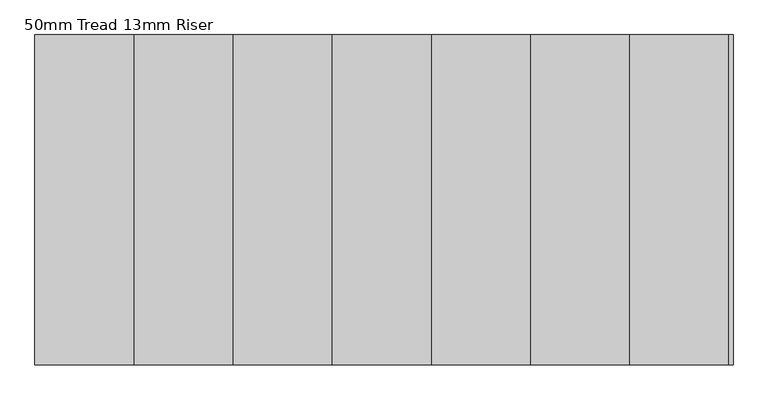
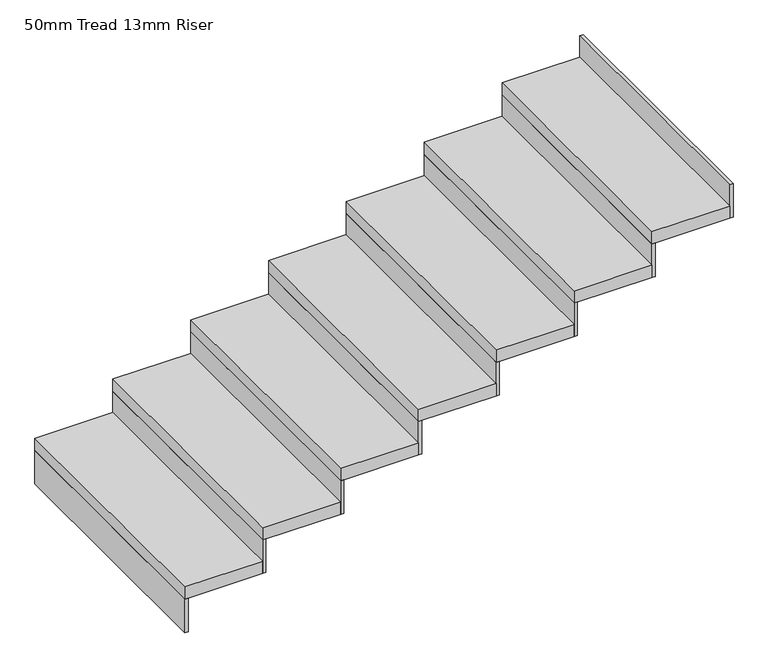
"""IFC4 building model written with IfcOpenShell, lengths in millimetres: stair flight geometry, 50mm Tread 13mm Riser."""

import ifcopenshell
import ifcopenshell.guid

model = None  # the IFC model being written
_history = None  # IfcOwnerHistory: only IFC2X3 demands one
_inside = {}  # id of a spatial element -> (the spatial element, [elements in it])
_under = {}  # id of a project, library or spatial element -> (it, [spatial elements below it])
_declared = {}  # id of a project -> (the project, [libraries it declares])
_typed = {}  # id of a type object -> (the type object, [elements of that type])
_made_of = {}  # id of a material, layer set ... -> (it, [elements and type objects made of it])


def new_model(schema):
    """Start an empty IFC model of exactly this schema.

    Asked for "IFC4X3", IfcOpenShell would pick the latest addendum, in which some entities
    have other attributes; the version numbers below select the first issue.
    IFC2X3 requires an IfcOwnerHistory on every rooted entity: one is made here for all.
    """
    global model, _history
    if schema == "IFC4X3":
        model = ifcopenshell.file(schema_version=(4, 3, 0, 0))
    else:
        model = ifcopenshell.file(schema=schema)
    _inside.clear()
    _under.clear()
    _declared.clear()
    _typed.clear()
    _made_of.clear()
    _history = None
    if model.schema == "IFC2X3":
        org = make("IfcOrganization", Name="unknown")
        user = make(
            "IfcPersonAndOrganization",
            ThePerson=make("IfcPerson", FamilyName="unknown"),
            TheOrganization=org,
        )
        app = make(
            "IfcApplication",
            ApplicationDeveloper=org,
            Version="unknown",
            ApplicationFullName="unknown",
            ApplicationIdentifier="unknown",
        )
        _history = make(
            "IfcOwnerHistory",
            OwningUser=user,
            OwningApplication=app,
            ChangeAction="ADDED",
            CreationDate=0,
        )
    return model


def make(cls, **values):
    """One entity of the class cls with the attributes given. An attribute that is None is left unset."""
    return model.create_entity(
        cls, **{name: value for name, value in values.items() if value is not None}
    )


def rooted(cls, **values):
    """An entity with a GlobalId (a new one), such as an element, a storey or a relation."""
    return make(cls, GlobalId=ifcopenshell.guid.new(), OwnerHistory=_history, **values)


def si_unit(unit_type, name, prefix=None):
    """IfcSIUnit, for example si_unit("LENGTHUNIT", "METRE", prefix="MILLI")."""
    return make("IfcSIUnit", UnitType=unit_type, Prefix=prefix, Name=name)


def assignment(units):
    """IfcUnitAssignment: the units of a project."""
    return None if units is None else make("IfcUnitAssignment", Units=units)


def point(xyz):
    """IfcCartesianPoint."""
    return None if xyz is None else make("IfcCartesianPoint", Coordinates=xyz)


def direction(xyz):
    """IfcDirection."""
    return None if xyz is None else make("IfcDirection", DirectionRatios=xyz)


def frame(location, z_axis=None, x_axis=None):
    """IfcAxis2Placement3D, a coordinate frame: its origin and axes. An axis left out is left unset."""
    return make(
        "IfcAxis2Placement3D",
        Location=point(location),
        Axis=direction(z_axis),
        RefDirection=direction(x_axis),
    )


def origin():
    """The frame at (0, 0, 0) with its axes left unset."""
    return frame((0.0, 0.0, 0.0))


def place(relative_to, where):
    """IfcLocalPlacement: puts the frame where relative to a parent placement (None: the world)."""
    return make(
        "IfcLocalPlacement", PlacementRelTo=relative_to, RelativePlacement=where
    )


def context(
    kind, dimensions, precision=None, world=None, true_north=None, identifier=None
):
    """IfcGeometricRepresentationContext, for example the 3D "Model" context."""
    return make(
        "IfcGeometricRepresentationContext",
        ContextIdentifier=identifier,
        ContextType=kind,
        CoordinateSpaceDimension=dimensions,
        Precision=precision,
        WorldCoordinateSystem=world,
        TrueNorth=true_north,
    )


def project(units=None, contexts=None):
    """IfcProject with its units and contexts."""
    return rooted(
        "IfcProject",
        Name="project",
        RepresentationContexts=contexts,
        UnitsInContext=assignment(units),
    )


def spatial(cls, under=None, at=None, **own):
    """A site, building, storey or space (cls), placed at a placement, below another one or the project."""
    s = rooted(cls, ObjectPlacement=at, **own)
    if under is not None:
        _under.setdefault(under.id(), (under, []))[1].append(s)
    return s


def polyline(points):
    """IfcPolyline through the points."""
    return make("IfcPolyline", Points=[point(p) for p in points])


def outline(outer, holes=None, kind="AREA"):
    """IfcArbitraryClosedProfileDef: a profile drawn as a closed curve; with holes, ...WithVoids."""
    if holes is None:
        return make("IfcArbitraryClosedProfileDef", ProfileType=kind, OuterCurve=outer)
    return make(
        "IfcArbitraryProfileDefWithVoids",
        ProfileType=kind,
        OuterCurve=outer,
        InnerCurves=holes,
    )


def extrude(swept, where, along, depth):
    """IfcExtrudedAreaSolid: the profile swept, set in the frame where, extruded along a direction by depth."""
    return make(
        "IfcExtrudedAreaSolid",
        SweptArea=swept,
        Position=where,
        ExtrudedDirection=direction(along),
        Depth=depth,
    )


def shape(context_of_items, identifier, shape_type, items):
    """IfcShapeRepresentation: the items that make up one representation, for example the "Body"."""
    return make(
        "IfcShapeRepresentation",
        ContextOfItems=context_of_items,
        RepresentationIdentifier=identifier,
        RepresentationType=shape_type,
        Items=items,
    )


def source(mapping_origin, context_of_items, identifier, shape_type, items):
    """IfcRepresentationMap: a shape defined once, which mapped items show again and again."""
    return make(
        "IfcRepresentationMap",
        MappingOrigin=mapping_origin,
        MappedRepresentation=shape(context_of_items, identifier, shape_type, items),
    )


def transform(
    local_origin,
    x_axis=None,
    y_axis=None,
    z_axis=None,
    scale=None,
    scale2=None,
    scale3=None,
    uniform=True,
):
    """IfcCartesianTransformationOperator3D, or its non-uniform kind. x_axis, y_axis, z_axis: its Axis1, 2, 3."""
    if uniform:
        return make(
            "IfcCartesianTransformationOperator3D",
            Axis1=direction(x_axis),
            Axis2=direction(y_axis),
            LocalOrigin=point(local_origin),
            Scale=scale,
            Axis3=direction(z_axis),
        )
    return make(
        "IfcCartesianTransformationOperator3DnonUniform",
        Axis1=direction(x_axis),
        Axis2=direction(y_axis),
        LocalOrigin=point(local_origin),
        Scale=scale,
        Axis3=direction(z_axis),
        Scale2=scale2,
        Scale3=scale3,
    )


def mapped(mapping_source, mapping_target):
    """IfcMappedItem: shows the shape of a source again, moved by a transform."""
    return make(
        "IfcMappedItem", MappingSource=mapping_source, MappingTarget=mapping_target
    )


def made_of(thing, what):
    """Note that an element or type object is made of a material, layer set ...; save() writes the relation."""
    if what is not None:
        _made_of.setdefault(what.id(), (what, []))[1].append(thing)
    return thing


def element(
    cls,
    number,
    at=None,
    inside=None,
    cuts=None,
    type_object=None,
    material=None,
    context=None,
    identifier="Body",
    shape_type=None,
    held_by="IfcProductDefinitionShape",
    body=None,
    shapes=None,
    **own,
):
    """One element of the class cls, such as IfcWall. Its Tag is "e" and its number.

    at: its placement. inside: the storey or other place that contains it. cuts: it is an
    opening in that element (IfcRelVoidsElement). A single representation is given by context,
    identifier, shape_type and body (its items); several are given by shapes. held_by: the class
    of the entity that holds the representations. save() writes the other relations.
    """
    e = rooted(cls, Tag="e%d" % number, ObjectPlacement=at, **own)
    if body is not None:
        shapes = [shape(context, identifier, shape_type, body)]
    if shapes is not None:
        e.Representation = make(held_by, Representations=shapes)
    if inside is not None:
        _inside.setdefault(inside.id(), (inside, []))[1].append(e)
    if cuts is not None:
        rooted(
            "IfcRelVoidsElement", RelatingBuildingElement=cuts, RelatedOpeningElement=e
        )
    if type_object is not None:
        _typed.setdefault(type_object.id(), (type_object, []))[1].append(e)
    return made_of(e, material)


def aggregate(whole, parts):
    """IfcRelAggregates: a whole, such as a stair, and the parts it consists of."""
    return rooted("IfcRelAggregates", RelatingObject=whole, RelatedObjects=parts)


def save(model, path):
    """Write the relations noted so far, then the file.

    IfcRelAggregates (storeys below a building ...), IfcRelContainedInSpatialStructure (elements
    in a storey), IfcRelDefinesByType, IfcRelAssociatesMaterial and IfcRelDeclares: one each for
    every whole, place, type object, material and project.
    """
    for whole, parts in _under.values():
        aggregate(whole, parts)
    for where, things in _inside.values():
        rooted(
            "IfcRelContainedInSpatialStructure",
            RelatedElements=things,
            RelatingStructure=where,
        )
    for kind, things in _typed.values():
        rooted("IfcRelDefinesByType", RelatedObjects=things, RelatingType=kind)
    for what, things in _made_of.values():
        rooted("IfcRelAssociatesMaterial", RelatedObjects=things, RelatingMaterial=what)
    for by, libraries in _declared.values():
        rooted("IfcRelDeclares", RelatingContext=by, RelatedDefinitions=libraries)
    model.write(path)


def stair_flight_50mm_tread_13mm_riser_0255b1fd(model_context):
    return source(origin(), model_context, "Body", "SweptSolid", [
        extrude(outline(polyline([(-12593.4172363, -3171.6396273), (-12605.9172363, -3171.6396273), (-12605.9172363, -2171.6396273), (-12593.4172363, -2171.6396273), (-12593.4172363, -3171.6396273)])), frame((0.0, 0.0, 1859.0909091), z_axis=(0.0, 0.0, 1.0), x_axis=(1.0, 0.0, 0.0)), (0.0, 0.0, 1.0), 136.3636364),
        extrude(outline(polyline([(-12305.9172363, -2171.6396273), (-12305.9172363, -3171.6396273), (-12605.9172363, -3171.6396273), (-12605.9172363, -2171.6396273), (-12305.9172363, -2171.6396273)])), frame((0.0, 0.0, 1995.4545455), z_axis=(0.0, 0.0, 1.0), x_axis=(1.0, 0.0, 0.0)), (0.0, 0.0, 1.0), 50.0),
        extrude(outline(polyline([(-12293.4172363, -3171.6396273), (-12305.9172363, -3171.6396273), (-12305.9172363, -2171.6396273), (-12293.4172363, -2171.6396273), (-12293.4172363, -3171.6396273)])), frame((0.0, 0.0, 1995.4545455), z_axis=(0.0, 0.0, 1.0), x_axis=(1.0, 0.0, 0.0)), (0.0, 0.0, 1.0), 136.3636364),
        extrude(outline(polyline([(-12005.9172363, -2171.6396273), (-12005.9172363, -3171.6396273), (-12305.9172363, -3171.6396273), (-12305.9172363, -2171.6396273), (-12005.9172363, -2171.6396273)])), frame((0.0, 0.0, 2131.8181818), z_axis=(0.0, 0.0, 1.0), x_axis=(1.0, 0.0, 0.0)), (0.0, 0.0, 1.0), 50.0),
        extrude(outline(polyline([(-11993.4172363, -3171.6396273), (-12005.9172363, -3171.6396273), (-12005.9172363, -2171.6396273), (-11993.4172363, -2171.6396273), (-11993.4172363, -3171.6396273)])), frame((0.0, 0.0, 2131.8181818), z_axis=(0.0, 0.0, 1.0), x_axis=(1.0, 0.0, 0.0)), (0.0, 0.0, 1.0), 136.3636364),
        extrude(outline(polyline([(-11705.9172363, -2171.6396273), (-11705.9172363, -3171.6396273), (-12005.9172363, -3171.6396273), (-12005.9172363, -2171.6396273), (-11705.9172363, -2171.6396273)])), frame((0.0, 0.0, 2268.1818182), z_axis=(0.0, 0.0, 1.0), x_axis=(1.0, 0.0, 0.0)), (0.0, 0.0, 1.0), 50.0),
        extrude(outline(polyline([(-11693.4172363, -3171.6396273), (-11705.9172363, -3171.6396273), (-11705.9172363, -2171.6396273), (-11693.4172363, -2171.6396273), (-11693.4172363, -3171.6396273)])), frame((0.0, 0.0, 2268.1818182), z_axis=(0.0, 0.0, 1.0), x_axis=(1.0, 0.0, 0.0)), (0.0, 0.0, 1.0), 136.3636364),
        extrude(outline(polyline([(-11405.9172363, -2171.6396273), (-11405.9172363, -3171.6396273), (-11705.9172363, -3171.6396273), (-11705.9172363, -2171.6396273), (-11405.9172363, -2171.6396273)])), frame((0.0, 0.0, 2404.5454545), z_axis=(0.0, 0.0, 1.0), x_axis=(1.0, 0.0, 0.0)), (0.0, 0.0, 1.0), 50.0),
        extrude(outline(polyline([(-11393.4172363, -3171.6396273), (-11405.9172363, -3171.6396273), (-11405.9172363, -2171.6396273), (-11393.4172363, -2171.6396273), (-11393.4172363, -3171.6396273)])), frame((0.0, 0.0, 2404.5454545), z_axis=(0.0, 0.0, 1.0), x_axis=(1.0, 0.0, 0.0)), (0.0, 0.0, 1.0), 136.3636364),
        extrude(outline(polyline([(-11105.9172363, -2171.6396273), (-11105.9172363, -3171.6396273), (-11405.9172363, -3171.6396273), (-11405.9172363, -2171.6396273), (-11105.9172363, -2171.6396273)])), frame((0.0, 0.0, 2540.9090909), z_axis=(0.0, 0.0, 1.0), x_axis=(1.0, 0.0, 0.0)), (0.0, 0.0, 1.0), 50.0),
        extrude(outline(polyline([(-11093.4172363, -3171.6396273), (-11105.9172363, -3171.6396273), (-11105.9172363, -2171.6396273), (-11093.4172363, -2171.6396273), (-11093.4172363, -3171.6396273)])), frame((0.0, 0.0, 2540.9090909), z_axis=(0.0, 0.0, 1.0), x_axis=(1.0, 0.0, 0.0)), (0.0, 0.0, 1.0), 136.3636364),
        extrude(outline(polyline([(-10805.9172363, -2171.6396273), (-10805.9172363, -3171.6396273), (-11105.9172363, -3171.6396273), (-11105.9172363, -2171.6396273), (-10805.9172363, -2171.6396273)])), frame((0.0, 0.0, 2677.2727273), z_axis=(0.0, 0.0, 1.0), x_axis=(1.0, 0.0, 0.0)), (0.0, 0.0, 1.0), 50.0),
        extrude(outline(polyline([(-10793.4172363, -3171.6396273), (-10805.9172363, -3171.6396273), (-10805.9172363, -2171.6396273), (-10793.4172363, -2171.6396273), (-10793.4172363, -3171.6396273)])), frame((0.0, 0.0, 2677.2727273), z_axis=(0.0, 0.0, 1.0), x_axis=(1.0, 0.0, 0.0)), (0.0, 0.0, 1.0), 136.3636364),
        extrude(outline(polyline([(-10505.9172363, -2171.6396273), (-10505.9172363, -3171.6396273), (-10805.9172363, -3171.6396273), (-10805.9172363, -2171.6396273), (-10505.9172363, -2171.6396273)])), frame((0.0, 0.0, 2813.6363636), z_axis=(0.0, 0.0, 1.0), x_axis=(1.0, 0.0, 0.0)), (0.0, 0.0, 1.0), 50.0),
        extrude(outline(polyline([(-10493.4172363, -3171.6396273), (-10505.9172363, -3171.6396273), (-10505.9172363, -2171.6396273), (-10493.4172363, -2171.6396273), (-10493.4172363, -3171.6396273)])), frame((0.0, 0.0, 2813.6363636), z_axis=(0.0, 0.0, 1.0), x_axis=(1.0, 0.0, 0.0)), (0.0, 0.0, 1.0), 136.3636364),
    ])


if __name__ == "__main__":
    model = new_model("IFC4")
    model_context = context("Model", 3, world=origin())
    ifc_project = project(units=[si_unit("LENGTHUNIT", "METRE", prefix="MILLI")], contexts=[model_context])
    site = spatial("IfcSite", under=ifc_project)
    building = spatial("IfcBuilding", under=site)
    placement = place(None, origin())
    stair_flight_50mm_tread_13mm_riser_shape = stair_flight_50mm_tread_13mm_riser_0255b1fd(model_context)
    element("IfcStairFlight", 1, ObjectType="50mm Tread 13mm Riser", at=placement, inside=building, context=model_context, shape_type="MappedRepresentation", body=[
        mapped(stair_flight_50mm_tread_13mm_riser_shape, transform((0.0, 0.0, 0.0), x_axis=(1.0, 0.0, 0.0), y_axis=(0.0, 1.0, 0.0), z_axis=(0.0, 0.0, 1.0))),
    ])
    save(model, "model.ifc")
